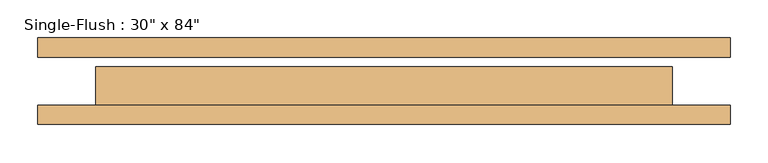
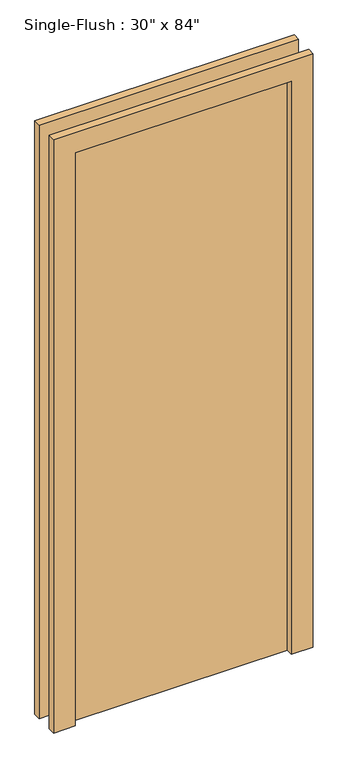
"""IFC4 building model written with IfcOpenShell, lengths in millimetres: door geometry."""

import ifcopenshell
import ifcopenshell.guid

model = None  # the IFC model being written
_history = None  # IfcOwnerHistory: only IFC2X3 demands one
_inside = {}  # id of a spatial element -> (the spatial element, [elements in it])
_under = {}  # id of a project, library or spatial element -> (it, [spatial elements below it])
_declared = {}  # id of a project -> (the project, [libraries it declares])
_typed = {}  # id of a type object -> (the type object, [elements of that type])
_made_of = {}  # id of a material, layer set ... -> (it, [elements and type objects made of it])


def new_model(schema):
    """Start an empty IFC model of exactly this schema.

    Asked for "IFC4X3", IfcOpenShell would pick the latest addendum, in which some entities
    have other attributes; the version numbers below select the first issue.
    IFC2X3 requires an IfcOwnerHistory on every rooted entity: one is made here for all.
    """
    global model, _history
    if schema == "IFC4X3":
        model = ifcopenshell.file(schema_version=(4, 3, 0, 0))
    else:
        model = ifcopenshell.file(schema=schema)
    _inside.clear()
    _under.clear()
    _declared.clear()
    _typed.clear()
    _made_of.clear()
    _history = None
    if model.schema == "IFC2X3":
        org = make("IfcOrganization", Name="unknown")
        user = make(
            "IfcPersonAndOrganization",
            ThePerson=make("IfcPerson", FamilyName="unknown"),
            TheOrganization=org,
        )
        app = make(
            "IfcApplication",
            ApplicationDeveloper=org,
            Version="unknown",
            ApplicationFullName="unknown",
            ApplicationIdentifier="unknown",
        )
        _history = make(
            "IfcOwnerHistory",
            OwningUser=user,
            OwningApplication=app,
            ChangeAction="ADDED",
            CreationDate=0,
        )
    return model


def make(cls, **values):
    """One entity of the class cls with the attributes given. An attribute that is None is left unset."""
    return model.create_entity(
        cls, **{name: value for name, value in values.items() if value is not None}
    )


def rooted(cls, **values):
    """An entity with a GlobalId (a new one), such as an element, a storey or a relation."""
    return make(cls, GlobalId=ifcopenshell.guid.new(), OwnerHistory=_history, **values)


def si_unit(unit_type, name, prefix=None):
    """IfcSIUnit, for example si_unit("LENGTHUNIT", "METRE", prefix="MILLI")."""
    return make("IfcSIUnit", UnitType=unit_type, Prefix=prefix, Name=name)


def assignment(units):
    """IfcUnitAssignment: the units of a project."""
    return None if units is None else make("IfcUnitAssignment", Units=units)


def point(xyz):
    """IfcCartesianPoint."""
    return None if xyz is None else make("IfcCartesianPoint", Coordinates=xyz)


def direction(xyz):
    """IfcDirection."""
    return None if xyz is None else make("IfcDirection", DirectionRatios=xyz)


def frame(location, z_axis=None, x_axis=None):
    """IfcAxis2Placement3D, a coordinate frame: its origin and axes. An axis left out is left unset."""
    return make(
        "IfcAxis2Placement3D",
        Location=point(location),
        Axis=direction(z_axis),
        RefDirection=direction(x_axis),
    )


def origin():
    """The frame at (0, 0, 0) with its axes left unset."""
    return frame((0.0, 0.0, 0.0))


def origin_with_axes():
    """The frame at (0, 0, 0) with the z axis (0, 0, 1) and the x axis (1, 0, 0) written out."""
    return frame((0.0, 0.0, 0.0), z_axis=(0.0, 0.0, 1.0), x_axis=(1.0, 0.0, 0.0))


def place(relative_to, where):
    """IfcLocalPlacement: puts the frame where relative to a parent placement (None: the world)."""
    return make(
        "IfcLocalPlacement", PlacementRelTo=relative_to, RelativePlacement=where
    )


def context(
    kind, dimensions, precision=None, world=None, true_north=None, identifier=None
):
    """IfcGeometricRepresentationContext, for example the 3D "Model" context."""
    return make(
        "IfcGeometricRepresentationContext",
        ContextIdentifier=identifier,
        ContextType=kind,
        CoordinateSpaceDimension=dimensions,
        Precision=precision,
        WorldCoordinateSystem=world,
        TrueNorth=true_north,
    )


def project(units=None, contexts=None):
    """IfcProject with its units and contexts."""
    return rooted(
        "IfcProject",
        Name="project",
        RepresentationContexts=contexts,
        UnitsInContext=assignment(units),
    )


def spatial(cls, under=None, at=None, **own):
    """A site, building, storey or space (cls), placed at a placement, below another one or the project."""
    s = rooted(cls, ObjectPlacement=at, **own)
    if under is not None:
        _under.setdefault(under.id(), (under, []))[1].append(s)
    return s


def polyline(points):
    """IfcPolyline through the points."""
    return make("IfcPolyline", Points=[point(p) for p in points])


def outline(outer, holes=None, kind="AREA"):
    """IfcArbitraryClosedProfileDef: a profile drawn as a closed curve; with holes, ...WithVoids."""
    if holes is None:
        return make("IfcArbitraryClosedProfileDef", ProfileType=kind, OuterCurve=outer)
    return make(
        "IfcArbitraryProfileDefWithVoids",
        ProfileType=kind,
        OuterCurve=outer,
        InnerCurves=holes,
    )


def extrude(swept, where, along, depth):
    """IfcExtrudedAreaSolid: the profile swept, set in the frame where, extruded along a direction by depth."""
    return make(
        "IfcExtrudedAreaSolid",
        SweptArea=swept,
        Position=where,
        ExtrudedDirection=direction(along),
        Depth=depth,
    )


def shape(context_of_items, identifier, shape_type, items):
    """IfcShapeRepresentation: the items that make up one representation, for example the "Body"."""
    return make(
        "IfcShapeRepresentation",
        ContextOfItems=context_of_items,
        RepresentationIdentifier=identifier,
        RepresentationType=shape_type,
        Items=items,
    )


def source(mapping_origin, context_of_items, identifier, shape_type, items):
    """IfcRepresentationMap: a shape defined once, which mapped items show again and again."""
    return make(
        "IfcRepresentationMap",
        MappingOrigin=mapping_origin,
        MappedRepresentation=shape(context_of_items, identifier, shape_type, items),
    )


def transform(
    local_origin,
    x_axis=None,
    y_axis=None,
    z_axis=None,
    scale=None,
    scale2=None,
    scale3=None,
    uniform=True,
):
    """IfcCartesianTransformationOperator3D, or its non-uniform kind. x_axis, y_axis, z_axis: its Axis1, 2, 3."""
    if uniform:
        return make(
            "IfcCartesianTransformationOperator3D",
            Axis1=direction(x_axis),
            Axis2=direction(y_axis),
            LocalOrigin=point(local_origin),
            Scale=scale,
            Axis3=direction(z_axis),
        )
    return make(
        "IfcCartesianTransformationOperator3DnonUniform",
        Axis1=direction(x_axis),
        Axis2=direction(y_axis),
        LocalOrigin=point(local_origin),
        Scale=scale,
        Axis3=direction(z_axis),
        Scale2=scale2,
        Scale3=scale3,
    )


def mapped(mapping_source, mapping_target):
    """IfcMappedItem: shows the shape of a source again, moved by a transform."""
    return make(
        "IfcMappedItem", MappingSource=mapping_source, MappingTarget=mapping_target
    )


def made_of(thing, what):
    """Note that an element or type object is made of a material, layer set ...; save() writes the relation."""
    if what is not None:
        _made_of.setdefault(what.id(), (what, []))[1].append(thing)
    return thing


def element(
    cls,
    number,
    at=None,
    inside=None,
    cuts=None,
    type_object=None,
    material=None,
    context=None,
    identifier="Body",
    shape_type=None,
    held_by="IfcProductDefinitionShape",
    body=None,
    shapes=None,
    **own,
):
    """One element of the class cls, such as IfcWall. Its Tag is "e" and its number.

    at: its placement. inside: the storey or other place that contains it. cuts: it is an
    opening in that element (IfcRelVoidsElement). A single representation is given by context,
    identifier, shape_type and body (its items); several are given by shapes. held_by: the class
    of the entity that holds the representations. save() writes the other relations.
    """
    e = rooted(cls, Tag="e%d" % number, ObjectPlacement=at, **own)
    if body is not None:
        shapes = [shape(context, identifier, shape_type, body)]
    if shapes is not None:
        e.Representation = make(held_by, Representations=shapes)
    if inside is not None:
        _inside.setdefault(inside.id(), (inside, []))[1].append(e)
    if cuts is not None:
        rooted(
            "IfcRelVoidsElement", RelatingBuildingElement=cuts, RelatedOpeningElement=e
        )
    if type_object is not None:
        _typed.setdefault(type_object.id(), (type_object, []))[1].append(e)
    return made_of(e, material)


def aggregate(whole, parts):
    """IfcRelAggregates: a whole, such as a stair, and the parts it consists of."""
    return rooted("IfcRelAggregates", RelatingObject=whole, RelatedObjects=parts)


def save(model, path):
    """Write the relations noted so far, then the file.

    IfcRelAggregates (storeys below a building ...), IfcRelContainedInSpatialStructure (elements
    in a storey), IfcRelDefinesByType, IfcRelAssociatesMaterial and IfcRelDeclares: one each for
    every whole, place, type object, material and project.
    """
    for whole, parts in _under.values():
        aggregate(whole, parts)
    for where, things in _inside.values():
        rooted(
            "IfcRelContainedInSpatialStructure",
            RelatedElements=things,
            RelatingStructure=where,
        )
    for kind, things in _typed.values():
        rooted("IfcRelDefinesByType", RelatedObjects=things, RelatingType=kind)
    for what, things in _made_of.values():
        rooted("IfcRelAssociatesMaterial", RelatedObjects=things, RelatingMaterial=what)
    for by, libraries in _declared.values():
        rooted("IfcRelDeclares", RelatingContext=by, RelatedDefinitions=libraries)
    model.write(path)


def door_8bc136cb(model_context):
    return source(origin(), model_context, "Body", "SweptSolid", [
        extrude(outline(polyline([(2209.8, -457.2), (0.0, -457.2), (0.0, -381.0), (2133.6, -381.0), (2133.6, 381.0), (0.0, 381.0), (0.0, 457.2), (2209.8, 457.2), (2209.8, -457.2)])), frame((0.0, -57.15, 0.0), z_axis=(0.0, 1.0, 0.0), x_axis=(0.0, 0.0, 1.0)), (0.0, 0.0, 1.0), 25.4),
        extrude(outline(polyline([(2209.8, 457.2), (2209.8, -457.2), (0.0, -457.2), (0.0, -381.0), (2133.6, -381.0), (2133.6, 381.0), (0.0, 381.0), (0.0, 457.2), (2209.8, 457.2)])), frame((0.0, 31.75, 0.0), z_axis=(0.0, 1.0, 0.0), x_axis=(0.0, 0.0, 1.0)), (0.0, 0.0, 1.0), 25.4),
        extrude(outline(polyline([(381.0, 19.05), (381.0, -31.75), (-381.0, -31.75), (-381.0, 19.05), (381.0, 19.05)])), origin_with_axes(), (0.0, 0.0, 1.0), 2133.6),
    ])


if __name__ == "__main__":
    model = new_model("IFC4")
    model_context = context("Model", 3, world=origin())
    ifc_project = project(units=[si_unit("LENGTHUNIT", "METRE", prefix="MILLI")], contexts=[model_context])
    site = spatial("IfcSite", under=ifc_project)
    building = spatial("IfcBuilding", under=site)
    placement = place(None, origin())
    door_shape = door_8bc136cb(model_context)
    element("IfcDoor", 1, ObjectType="Single-Flush : 30\" x 84\"", at=placement, inside=building, context=model_context, shape_type="MappedRepresentation", body=[
        mapped(door_shape, transform((0.0, 0.0, 0.0), x_axis=(1.0, 0.0, 0.0), y_axis=(0.0, 1.0, 0.0), z_axis=(0.0, 0.0, 1.0))),
    ])
    save(model, "model.ifc")

# Revit data of these elements
# Type "Single-Flush : 30\" x 84\""
#   Type Mark = "4"
#   Construction Type Id = "MDOOR"
#   Assembly Code = "C1020"
#   Analytic Construction = "Metal"
#   Thickness = 0' - 2"
#   Heat Transfer Coefficient (U) = 0.651978 BTU/(h·ft²·°F)
#   Height = 7' - 0"
#   Trim Projection Ext = 0' - 1"
#   Trim Projection Int = 0' - 1"
#   Trim Width = 0' - 3"
#   Width = 2' - 6"
#   Define Thermal Properties by = 1
#   Define Thermal Properties by = 1
#   Door Material = Door - Panel
#   Frame Material = Door - Frame
#   Visual Light Transmittance = 0
#   Solar Heat Gain Coefficient = 0
#   Function = (empty or 0)
#   Wall Closure = (empty or 0)
# Element 1 (IfcDoor, "Single-Flush : 30\" x 84\"")
#   Materials on its faces: "Door - Frame", "Door - Panel"
# Materials
#   "Door - Panel": class "Wood", colour RGB 210 159 95, transparency 0, Cost = 0
#   "Door - Frame": class "Miscellaneous", colour RGB 118 70 51, transparency 0, Cost = 0
